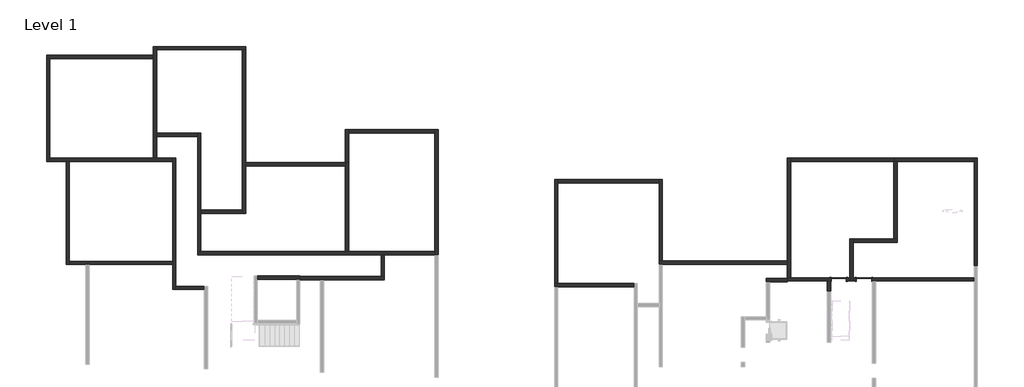
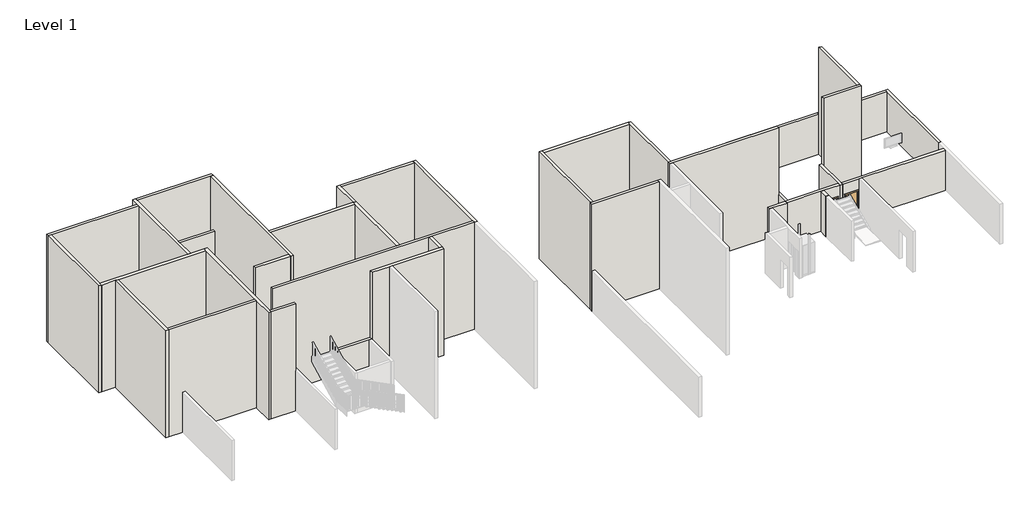
# One storey, part 2 of 3: 38 walls, 2 doors.
"""IFC4 building model written with IfcOpenShell, lengths in millimetres."""

import ifcopenshell
import ifcopenshell.guid

model = None  # the IFC model being written
_history = None  # IfcOwnerHistory: only IFC2X3 demands one
_inside = {}  # id of a spatial element -> (the spatial element, [elements in it])
_under = {}  # id of a project, library or spatial element -> (it, [spatial elements below it])
_declared = {}  # id of a project -> (the project, [libraries it declares])
_typed = {}  # id of a type object -> (the type object, [elements of that type])
_made_of = {}  # id of a material, layer set ... -> (it, [elements and type objects made of it])


def new_model(schema):
    """Start an empty IFC model of exactly this schema.

    Asked for "IFC4X3", IfcOpenShell would pick the latest addendum, in which some entities
    have other attributes; the version numbers below select the first issue.
    IFC2X3 requires an IfcOwnerHistory on every rooted entity: one is made here for all.
    """
    global model, _history
    if schema == "IFC4X3":
        model = ifcopenshell.file(schema_version=(4, 3, 0, 0))
    else:
        model = ifcopenshell.file(schema=schema)
    _inside.clear()
    _under.clear()
    _declared.clear()
    _typed.clear()
    _made_of.clear()
    _history = None
    if model.schema == "IFC2X3":
        org = make("IfcOrganization", Name="unknown")
        user = make(
            "IfcPersonAndOrganization",
            ThePerson=make("IfcPerson", FamilyName="unknown"),
            TheOrganization=org,
        )
        app = make(
            "IfcApplication",
            ApplicationDeveloper=org,
            Version="unknown",
            ApplicationFullName="unknown",
            ApplicationIdentifier="unknown",
        )
        _history = make(
            "IfcOwnerHistory",
            OwningUser=user,
            OwningApplication=app,
            ChangeAction="ADDED",
            CreationDate=0,
        )
    return model


def make(cls, **values):
    """One entity of the class cls with the attributes given. An attribute that is None is left unset."""
    return model.create_entity(
        cls, **{name: value for name, value in values.items() if value is not None}
    )


def rooted(cls, **values):
    """An entity with a GlobalId (a new one), such as an element, a storey or a relation."""
    return make(cls, GlobalId=ifcopenshell.guid.new(), OwnerHistory=_history, **values)


def si_unit(unit_type, name, prefix=None):
    """IfcSIUnit, for example si_unit("LENGTHUNIT", "METRE", prefix="MILLI")."""
    return make("IfcSIUnit", UnitType=unit_type, Prefix=prefix, Name=name)


def assignment(units):
    """IfcUnitAssignment: the units of a project."""
    return None if units is None else make("IfcUnitAssignment", Units=units)


def point(xyz):
    """IfcCartesianPoint."""
    return None if xyz is None else make("IfcCartesianPoint", Coordinates=xyz)


def direction(xyz):
    """IfcDirection."""
    return None if xyz is None else make("IfcDirection", DirectionRatios=xyz)


def frame(location, z_axis=None, x_axis=None):
    """IfcAxis2Placement3D, a coordinate frame: its origin and axes. An axis left out is left unset."""
    return make(
        "IfcAxis2Placement3D",
        Location=point(location),
        Axis=direction(z_axis),
        RefDirection=direction(x_axis),
    )


def origin():
    """The frame at (0, 0, 0) with its axes left unset."""
    return frame((0.0, 0.0, 0.0))


def origin_with_axes():
    """The frame at (0, 0, 0) with the z axis (0, 0, 1) and the x axis (1, 0, 0) written out."""
    return frame((0.0, 0.0, 0.0), z_axis=(0.0, 0.0, 1.0), x_axis=(1.0, 0.0, 0.0))


def place(relative_to, where):
    """IfcLocalPlacement: puts the frame where relative to a parent placement (None: the world)."""
    return make(
        "IfcLocalPlacement", PlacementRelTo=relative_to, RelativePlacement=where
    )


def context(
    kind, dimensions, precision=None, world=None, true_north=None, identifier=None
):
    """IfcGeometricRepresentationContext, for example the 3D "Model" context."""
    return make(
        "IfcGeometricRepresentationContext",
        ContextIdentifier=identifier,
        ContextType=kind,
        CoordinateSpaceDimension=dimensions,
        Precision=precision,
        WorldCoordinateSystem=world,
        TrueNorth=true_north,
    )


def project(units=None, contexts=None):
    """IfcProject with its units and contexts."""
    return rooted(
        "IfcProject",
        Name="project",
        RepresentationContexts=contexts,
        UnitsInContext=assignment(units),
    )


def spatial(cls, under=None, at=None, **own):
    """A site, building, storey or space (cls), placed at a placement, below another one or the project."""
    s = rooted(cls, ObjectPlacement=at, **own)
    if under is not None:
        _under.setdefault(under.id(), (under, []))[1].append(s)
    return s


def polyline(points):
    """IfcPolyline through the points."""
    return make("IfcPolyline", Points=[point(p) for p in points])


def outline(outer, holes=None, kind="AREA"):
    """IfcArbitraryClosedProfileDef: a profile drawn as a closed curve; with holes, ...WithVoids."""
    if holes is None:
        return make("IfcArbitraryClosedProfileDef", ProfileType=kind, OuterCurve=outer)
    return make(
        "IfcArbitraryProfileDefWithVoids",
        ProfileType=kind,
        OuterCurve=outer,
        InnerCurves=holes,
    )


def extrude(swept, where, along, depth):
    """IfcExtrudedAreaSolid: the profile swept, set in the frame where, extruded along a direction by depth."""
    return make(
        "IfcExtrudedAreaSolid",
        SweptArea=swept,
        Position=where,
        ExtrudedDirection=direction(along),
        Depth=depth,
    )


def faces_of(points, faces, orient=None, outer=None):
    """IfcFace entities. A face is a list of loops; a loop is a list of indices into points, from 0.

    orient and outer hold one flag for each loop. By default every Orientation is true, the
    first loop of a face is its IfcFaceOuterBound and the others are IfcFaceBound.
    """
    made = []
    for i, loops in enumerate(faces):
        bounds = []
        for j, loop in enumerate(loops):
            is_outer = j == 0 if outer is None else outer[i][j]
            bounds.append(
                make(
                    "IfcFaceOuterBound" if is_outer else "IfcFaceBound",
                    Bound=make("IfcPolyLoop", Polygon=[points[k] for k in loop]),
                    Orientation=True if orient is None else orient[i][j],
                )
            )
        made.append(make("IfcFace", Bounds=bounds))
    return made


def faceted_brep(points, faces, orient=None, outer=None, voids=None):
    """IfcFacetedBrep: a solid bounded by flat faces; with voids (closed shells), ...WithVoids."""
    shared = [point(p) for p in points]
    hull = make("IfcClosedShell", CfsFaces=faces_of(shared, faces, orient, outer))
    if voids is None:
        return make("IfcFacetedBrep", Outer=hull)
    return make(
        "IfcFacetedBrepWithVoids",
        Outer=hull,
        Voids=[
            make(cls, CfsFaces=faces_of(shared, fs, o, b)) for cls, fs, o, b in voids
        ],
    )


def shape(context_of_items, identifier, shape_type, items):
    """IfcShapeRepresentation: the items that make up one representation, for example the "Body"."""
    return make(
        "IfcShapeRepresentation",
        ContextOfItems=context_of_items,
        RepresentationIdentifier=identifier,
        RepresentationType=shape_type,
        Items=items,
    )


def source(mapping_origin, context_of_items, identifier, shape_type, items):
    """IfcRepresentationMap: a shape defined once, which mapped items show again and again."""
    return make(
        "IfcRepresentationMap",
        MappingOrigin=mapping_origin,
        MappedRepresentation=shape(context_of_items, identifier, shape_type, items),
    )


def transform(
    local_origin,
    x_axis=None,
    y_axis=None,
    z_axis=None,
    scale=None,
    scale2=None,
    scale3=None,
    uniform=True,
):
    """IfcCartesianTransformationOperator3D, or its non-uniform kind. x_axis, y_axis, z_axis: its Axis1, 2, 3."""
    if uniform:
        return make(
            "IfcCartesianTransformationOperator3D",
            Axis1=direction(x_axis),
            Axis2=direction(y_axis),
            LocalOrigin=point(local_origin),
            Scale=scale,
            Axis3=direction(z_axis),
        )
    return make(
        "IfcCartesianTransformationOperator3DnonUniform",
        Axis1=direction(x_axis),
        Axis2=direction(y_axis),
        LocalOrigin=point(local_origin),
        Scale=scale,
        Axis3=direction(z_axis),
        Scale2=scale2,
        Scale3=scale3,
    )


def mapped(mapping_source, mapping_target):
    """IfcMappedItem: shows the shape of a source again, moved by a transform."""
    return make(
        "IfcMappedItem", MappingSource=mapping_source, MappingTarget=mapping_target
    )


def made_of(thing, what):
    """Note that an element or type object is made of a material, layer set ...; save() writes the relation."""
    if what is not None:
        _made_of.setdefault(what.id(), (what, []))[1].append(thing)
    return thing


def element(
    cls,
    number,
    at=None,
    inside=None,
    cuts=None,
    type_object=None,
    material=None,
    context=None,
    identifier="Body",
    shape_type=None,
    held_by="IfcProductDefinitionShape",
    body=None,
    shapes=None,
    **own,
):
    """One element of the class cls, such as IfcWall. Its Tag is "e" and its number.

    at: its placement. inside: the storey or other place that contains it. cuts: it is an
    opening in that element (IfcRelVoidsElement). A single representation is given by context,
    identifier, shape_type and body (its items); several are given by shapes. held_by: the class
    of the entity that holds the representations. save() writes the other relations.
    """
    e = rooted(cls, Tag="e%d" % number, ObjectPlacement=at, **own)
    if body is not None:
        shapes = [shape(context, identifier, shape_type, body)]
    if shapes is not None:
        e.Representation = make(held_by, Representations=shapes)
    if inside is not None:
        _inside.setdefault(inside.id(), (inside, []))[1].append(e)
    if cuts is not None:
        rooted(
            "IfcRelVoidsElement", RelatingBuildingElement=cuts, RelatedOpeningElement=e
        )
    if type_object is not None:
        _typed.setdefault(type_object.id(), (type_object, []))[1].append(e)
    return made_of(e, material)


def aggregate(whole, parts):
    """IfcRelAggregates: a whole, such as a stair, and the parts it consists of."""
    return rooted("IfcRelAggregates", RelatingObject=whole, RelatedObjects=parts)


def save(model, path):
    """Write the relations noted so far, then the file.

    IfcRelAggregates (storeys below a building ...), IfcRelContainedInSpatialStructure (elements
    in a storey), IfcRelDefinesByType, IfcRelAssociatesMaterial and IfcRelDeclares: one each for
    every whole, place, type object, material and project.
    """
    for whole, parts in _under.values():
        aggregate(whole, parts)
    for where, things in _inside.values():
        rooted(
            "IfcRelContainedInSpatialStructure",
            RelatedElements=things,
            RelatingStructure=where,
        )
    for kind, things in _typed.values():
        rooted("IfcRelDefinesByType", RelatedObjects=things, RelatingType=kind)
    for what, things in _made_of.values():
        rooted("IfcRelAssociatesMaterial", RelatedObjects=things, RelatingMaterial=what)
    for by, libraries in _declared.values():
        rooted("IfcRelDeclares", RelatingContext=by, RelatedDefinitions=libraries)
    model.write(path)


def m_single_flush_0915_x_2134mm_727434cd(model_context):
    return source(origin(), model_context, "Body", "SweptSolid", [
        extrude(outline(polyline([(2210.0, -533.5), (0.0, -533.5), (0.0, -457.5), (2134.0, -457.5), (2134.0, 457.5), (0.0, 457.5), (0.0, 533.5), (2210.0, 533.5), (2210.0, -533.5)])), frame((0.0, -125.0, 0.0), z_axis=(0.0, 1.0, 0.0), x_axis=(0.0, 0.0, 1.0)), (0.0, 0.0, 1.0), 25.0),
        extrude(outline(polyline([(2210.0, 533.5), (2210.0, -533.5), (0.0, -533.5), (0.0, -457.5), (2134.0, -457.5), (2134.0, 457.5), (0.0, 457.5), (0.0, 533.5), (2210.0, 533.5)])), frame((0.0, 100.0, 0.0), z_axis=(0.0, 1.0, 0.0), x_axis=(0.0, 0.0, 1.0)), (0.0, 0.0, 1.0), 25.0),
        extrude(outline(polyline([(457.5, -49.0), (457.5, -100.0), (-457.5, -100.0), (-457.5, -49.0), (457.5, -49.0)])), origin_with_axes(), (0.0, 0.0, 1.0), 2134.0),
    ])


def m_single_flush_0915_x_2134mm_6a9e8738(model_context):
    return source(origin(), model_context, "Body", "SweptSolid", [
        extrude(outline(polyline([(2210.0, -533.5), (0.0, -533.5), (0.0, -457.5), (2134.0, -457.5), (2134.0, 457.5), (0.0, 457.5), (0.0, 533.5), (2210.0, 533.5), (2210.0, -533.5)])), frame((0.0, 100.0, 0.0), z_axis=(0.0, 1.0, 0.0), x_axis=(0.0, 0.0, 1.0)), (0.0, 0.0, 1.0), 25.0),
        extrude(outline(polyline([(2210.0, 533.5), (2210.0, -533.5), (0.0, -533.5), (0.0, -457.5), (2134.0, -457.5), (2134.0, 457.5), (0.0, 457.5), (0.0, 533.5), (2210.0, 533.5)])), frame((0.0, -125.0, 0.0), z_axis=(0.0, 1.0, 0.0), x_axis=(0.0, 0.0, 1.0)), (0.0, 0.0, 1.0), 25.0),
        extrude(outline(polyline([(457.5, 49.0), (-457.5, 49.0), (-457.5, 100.0), (457.5, 100.0), (457.5, 49.0)])), origin_with_axes(), (0.0, 0.0, 1.0), 2134.0),
    ])


model = new_model("IFC4")

# Units and contexts
model_context = context("Model", 3, world=origin())
ifc_project = project(units=[si_unit("LENGTHUNIT", "METRE", prefix="MILLI")], contexts=[model_context])

# Site, building, storey
site = spatial("IfcSite", under=ifc_project)
building = spatial("IfcBuilding", under=site)
storey = spatial("IfcBuildingStorey", under=building, Name="Level 1", Elevation=0.0)

# Doors
placement = place(None, origin())
m_single_flush_0915_x_2134mm_shape = m_single_flush_0915_x_2134mm_727434cd(model_context)
element("IfcDoor", 1, ObjectType="M_Single-Flush : 0915 x 2134mm", at=placement, inside=storey, context=model_context, shape_type="MappedRepresentation", body=[
    mapped(m_single_flush_0915_x_2134mm_shape, transform((23447.336337, 519.475628, 0.0), x_axis=(-1.0, 0.0, 0.0), y_axis=(0.0, -1.0, 0.0), z_axis=(0.0, 0.0, 1.0))),
])
m_single_flush_0915_x_2134mm_2_shape = m_single_flush_0915_x_2134mm_6a9e8738(model_context)
element("IfcDoor", 2, ObjectType="M_Single-Flush : 0915 x 2134mm", at=placement, inside=storey, context=model_context, shape_type="MappedRepresentation", body=[
    mapped(m_single_flush_0915_x_2134mm_2_shape, transform((21932.336337, 519.475628, 0.0), x_axis=(1.0, 0.0, 0.0), y_axis=(0.0, 1.0, 0.0), z_axis=(0.0, 0.0, 1.0))),
])

# Walls
element("IfcWall", 3, ObjectType="Generic - 200mm", at=placement, inside=storey, context=model_context, shape_type="Brep", body=[
    faceted_brep([(25249.836337, 7619.475628, 0.0), (25449.836337, 7619.475628, 0.0), (30068.3425199, 7619.475628, 0.0), (30068.3425199, 7619.475628, 3000.0), (25249.836337, 7619.475628, 3000.0), (25249.836337, 7819.475628, 0.0), (25249.836337, 7819.475628, 3000.0), (30068.3425199, 7819.475628, 3000.0), (30068.3425199, 7819.475628, 0.0)], [[[0, 1, 2, 3, 4]], [[5, 6, 7, 8]], [[2, 1, 0, 5, 8]], [[4, 3, 7, 6]], [[3, 2, 8, 7]], [[0, 4, 6, 5]]]),
])
element("IfcWall", 4, ObjectType="Generic - 200mm", at=placement, inside=storey, context=model_context, shape_type="Brep", body=[
    faceted_brep([(30068.3425199, 7819.475628, 0.0), (30068.3425199, 7619.475628, 0.0), (30068.3425199, 1319.475628, 0.0), (30068.3425199, 1319.475628, 3000.0), (30068.3425199, 7619.475628, 3000.0), (30068.3425199, 7819.475628, 3000.0), (30268.3425199, 7819.475628, 0.0), (30268.3425199, 7819.475628, 3000.0), (30268.3425199, 1319.475628, 3000.0), (30268.3425199, 1319.475628, 0.0), (30068.8612349, 1319.475628, 0.0), (30068.8612349, 1319.475628, 3000.0)], [[[0, 1, 2, 3, 4, 5]], [[6, 7, 8, 9]], [[2, 1, 0, 6, 9, 10]], [[3, 2, 10, 9, 8, 11]], [[5, 4, 3, 11, 8, 7]], [[0, 5, 7, 6]]]),
])
element("IfcWall", 5, ObjectType="Generic - 200mm", at=placement, inside=storey, context=model_context, shape_type="SweptSolid", body=[
    extrude(outline(polyline([(21449.836337, 419.475628), (21449.836337, -200.524372), (21249.836337, -200.524372), (21249.836337, 419.475628), (21449.836337, 419.475628)])), origin_with_axes(), (0.0, 0.0, 1.0), 3000.0),
])
element("IfcWall", 6, ObjectType="Generic - 200mm", at=placement, inside=storey, context=model_context, shape_type="SweptSolid", body=[
    extrude(outline(polyline([(25249.836337, 7619.475628), (19028.8612349, 7619.475628), (19028.8612349, 7819.475628), (25249.836337, 7819.475628), (25249.836337, 7619.475628)])), origin_with_axes(), (0.0, 0.0, 1.0), 3000.0),
])
element("IfcWall", 7, ObjectType="Generic - 200mm", at=placement, inside=storey, context=model_context, shape_type="Brep", body=[
    faceted_brep([(22789.836337, 419.475628, 0.0), (22789.836337, 619.475628, 0.0), (22789.836337, 2754.475628, 0.0), (22789.836337, 2954.475628, 0.0), (22789.836337, 2954.475628, 3000.0), (22789.836337, 619.475628, 3000.0), (22789.836337, 419.475628, 3000.0), (22589.836337, 419.475628, 0.0), (22589.836337, 419.475628, 3000.0), (22589.836337, 619.475628, 3000.0), (22589.836337, 2954.475628, 3000.0), (22589.836337, 2954.475628, 0.0), (22589.836337, 619.475628, 0.0)], [[[0, 1, 2, 3, 4, 5, 6]], [[7, 8, 9, 10, 11, 12]], [[3, 2, 1, 0, 7, 12, 11]], [[6, 5, 4, 10, 9, 8]], [[0, 6, 8, 7]], [[4, 3, 11, 10]]]),
])
element("IfcWall", 8, ObjectType="Generic - 200mm", at=placement, inside=storey, context=model_context, shape_type="Brep", body=[
    faceted_brep([(18828.8612349, 7819.475628, 0.0), (18828.8612349, 1619.475628, 0.0), (18828.8612349, 1419.475628, 0.0), (18828.8612349, 619.475628, 0.0), (18828.8612349, 619.475628, 3000.0), (18828.8612349, 7819.475628, 3000.0), (19028.8612349, 7819.475628, 0.0), (19028.8612349, 7819.475628, 3000.0), (19028.8612349, 7619.475628, 3000.0), (19028.8612349, 619.475628, 3000.0), (19028.8612349, 619.475628, 0.0), (19028.8612349, 7619.475628, 0.0)], [[[0, 1, 2, 3, 4, 5]], [[6, 7, 8, 9, 10, 11]], [[3, 2, 1, 0, 6, 11, 10]], [[5, 4, 9, 8, 7]], [[4, 3, 10, 9]], [[0, 5, 7, 6]]]),
])
element("IfcWall", 9, ObjectType="Generic - 200mm", at=placement, inside=storey, context=model_context, shape_type="Brep", body=[
    faceted_brep([(30068.8612349, 419.475628, 3000.0), (24148.8612349, 419.475628, 3000.0), (23948.8612349, 419.475628, 3000.0), (22789.836337, 419.475628, 3000.0), (22789.836337, 419.475628, 0.0), (22989.836337, 419.475628, 0.0), (22989.836337, 419.475628, 2134.0), (23904.836337, 419.475628, 2134.0), (23904.836337, 419.475628, 0.0), (23948.8612349, 419.475628, 0.0), (24148.8612349, 419.475628, 0.0), (30068.8612349, 419.475628, 0.0), (22789.836337, 619.475628, 3000.0), (30068.8612349, 619.475628, 3000.0), (30068.8612349, 619.475628, 0.0), (23904.836337, 619.475628, 0.0), (23904.836337, 619.475628, 2134.0), (22989.836337, 619.475628, 2134.0), (22989.836337, 619.475628, 0.0), (22789.836337, 619.475628, 0.0)], [[[0, 1, 2, 3, 4, 5, 6, 7, 8, 9, 10, 11]], [[12, 13, 14, 15, 16, 17, 18, 19]], [[14, 11, 10, 9, 8, 15]], [[4, 19, 18, 5]], [[3, 2, 1, 0, 13, 12]], [[0, 11, 14, 13]], [[4, 3, 12, 19]], [[17, 6, 5, 18]], [[7, 16, 15, 8]], [[16, 7, 6, 17]]]),
])
element("IfcWall", 10, ObjectType="Generic - 200mm", at=placement, inside=storey, context=model_context, shape_type="Brep", body=[
    faceted_brep([(18828.8612349, 579.475628, 0.0), (17570.6041014, 579.475628, 0.0), (17570.6041014, 579.475628, 3000.0), (18828.8612349, 579.475628, 3000.0), (18828.8612349, 379.475628, 0.0), (18828.8612349, 379.475628, 3000.0), (17770.6041014, 379.475628, 3000.0), (17570.6041014, 379.475628, 3000.0), (17570.6041014, 379.475628, 0.0), (17770.6041014, 379.475628, 0.0), (18828.8612349, 419.475628, 0.0), (18828.8612349, 419.475628, 3000.0)], [[[0, 1, 2, 3]], [[4, 5, 6, 7, 8, 9]], [[1, 0, 10, 4, 9, 8]], [[2, 1, 8, 7]], [[3, 2, 7, 6, 5, 11]], [[0, 3, 11, 5, 4, 10]]]),
])
element("IfcWall", 11, ObjectType="Generic - 200mm", at=placement, inside=storey, context=model_context, shape_type="Brep", body=[
    faceted_brep([(18828.8612349, 619.475628, 3000.0), (19028.8612349, 619.475628, 3000.0), (22589.836337, 619.475628, 3000.0), (22589.836337, 619.475628, 0.0), (22389.836337, 619.475628, 0.0), (22389.836337, 619.475628, 2134.0), (21474.836337, 619.475628, 2134.0), (21474.836337, 619.475628, 0.0), (19028.8612349, 619.475628, 0.0), (18828.8612349, 619.475628, 0.0), (22589.836337, 419.475628, 3000.0), (21449.836337, 419.475628, 3000.0), (21249.836337, 419.475628, 3000.0), (18828.8612349, 419.475628, 3000.0), (18828.8612349, 419.475628, 0.0), (21249.836337, 419.475628, 0.0), (21449.836337, 419.475628, 0.0), (21474.836337, 419.475628, 0.0), (21474.836337, 419.475628, 2134.0), (22389.836337, 419.475628, 2134.0), (22389.836337, 419.475628, 0.0), (22589.836337, 419.475628, 0.0), (18828.8612349, 579.475628, 0.0), (18828.8612349, 579.475628, 3000.0)], [[[0, 1, 2, 3, 4, 5, 6, 7, 8, 9]], [[10, 11, 12, 13, 14, 15, 16, 17, 18, 19, 20, 21]], [[3, 21, 20, 4]], [[14, 22, 9, 8, 7, 17, 16, 15]], [[2, 1, 0, 23, 13, 12, 11, 10]], [[0, 9, 22, 14, 13, 23]], [[3, 2, 10, 21]], [[19, 5, 4, 20]], [[6, 18, 17, 7]], [[18, 6, 5, 19]]]),
])
element("IfcWall", 12, ObjectType="Generic - 200mm", at=placement, inside=storey, context=model_context, shape_type="Brep", body=[
    faceted_brep([(22789.836337, 2754.475628, 0.0), (25449.836337, 2754.475628, 0.0), (25449.836337, 2754.475628, 8000.0), (22789.836337, 2754.475628, 8000.0), (22789.836337, 2954.475628, 0.0), (22789.836337, 2954.475628, 3000.0), (22789.836337, 2954.475628, 8000.0), (25249.836337, 2954.475628, 8000.0), (25449.836337, 2954.475628, 8000.0), (25449.836337, 2954.475628, 0.0), (25249.836337, 2954.475628, 0.0)], [[[0, 1, 2, 3]], [[4, 5, 6, 7, 8, 9, 10]], [[1, 0, 4, 10, 9]], [[3, 2, 8, 7, 6]], [[2, 1, 9, 8]], [[0, 3, 6, 5, 4]]]),
])
element("IfcWall", 13, ObjectType="Generic - 200mm", at=placement, inside=storey, context=model_context, shape_type="Brep", body=[
    faceted_brep([(25449.836337, 2954.475628, 0.0), (25449.836337, 7619.475628, 0.0), (25449.836337, 7619.475628, 8000.0), (25449.836337, 2954.475628, 8000.0), (25249.836337, 2954.475628, 0.0), (25249.836337, 2954.475628, 8000.0), (25249.836337, 7619.475628, 8000.0), (25249.836337, 7619.475628, 3000.0), (25249.836337, 7619.475628, 0.0)], [[[0, 1, 2, 3]], [[4, 5, 6, 7, 8]], [[1, 0, 4, 8]], [[3, 2, 6, 5]], [[0, 3, 5, 4]], [[2, 1, 8, 7, 6]]]),
])
element("IfcWall", 14, ObjectType="Generic - 200mm", at=placement, inside=storey, context=model_context, shape_type="Brep", body=[
    faceted_brep([(-10469.8304233, 720.8372871, 0.0), (-13026.101437, 720.8372871, 0.0), (-13026.101437, 720.8372871, 3000.0), (-10469.8304233, 720.8372871, 3000.0), (-10469.8304233, 520.8372871, 0.0), (-10469.8304233, 520.8372871, 3000.0), (-10669.8304233, 520.8372871, 3000.0), (-13026.101437, 520.8372871, 3000.0), (-13026.101437, 520.8372871, 0.0), (-10669.8304233, 520.8372871, 0.0), (-10469.8304233, 700.8372871, 0.0)], [[[0, 1, 2, 3]], [[4, 5, 6, 7, 8, 9]], [[1, 0, 10, 4, 9, 8]], [[3, 2, 7, 6, 5]], [[2, 1, 8, 7]], [[0, 3, 5, 4, 10]]]),
])
element("IfcWall", 15, ObjectType="Generic - 200mm", at=placement, inside=storey, context=model_context, shape_type="Brep", body=[
    faceted_brep([(-19089.8304233, 7812.8400285, 0.0), (-19089.8304233, 9112.8400285, 0.0), (-19089.8304233, 9312.8400285, 0.0), (-19089.8304233, 14340.8372871, 0.0), (-19089.8304233, 14540.8372871, 0.0), (-19089.8304233, 14540.8372871, 8000.0), (-19089.8304233, 14340.8372871, 8000.0), (-19089.8304233, 9312.8400285, 8000.0), (-19089.8304233, 9112.8400285, 8000.0), (-19089.8304233, 7812.8400285, 8000.0), (-19289.8304233, 7812.8400285, 0.0), (-19289.8304233, 7812.8400285, 8000.0), (-19289.8304233, 13812.8400285, 8000.0), (-19289.8304233, 14012.8400285, 8000.0), (-19289.8304233, 14540.8372871, 8000.0), (-19289.8304233, 14540.8372871, 0.0), (-19289.8304233, 14012.8400285, 0.0), (-19289.8304233, 13812.8400285, 0.0)], [[[0, 1, 2, 3, 4, 5, 6, 7, 8, 9]], [[10, 11, 12, 13, 14, 15, 16, 17]], [[4, 3, 2, 1, 0, 10, 17, 16, 15]], [[9, 8, 7, 6, 5, 14, 13, 12, 11]], [[5, 4, 15, 14]], [[0, 9, 11, 10]]]),
])
element("IfcWall", 16, ObjectType="Generic - 200mm", at=placement, inside=storey, context=model_context, shape_type="Brep", body=[
    faceted_brep([(9628.8612349, 279.9901881, 0.0), (5043.716007, 279.9901881, 0.0), (4843.716007, 279.9901881, 0.0), (4843.716007, 279.9901881, 8000.0), (5043.716007, 279.9901881, 8000.0), (9628.8612349, 279.9901881, 8000.0), (9628.8612349, 79.9901881, 0.0), (9628.8612349, 79.9901881, 8000.0), (4843.716007, 79.9901881, 8000.0), (4843.716007, 79.9901881, 3000.0), (4843.716007, 79.9901881, 0.0), (5043.716007, 79.9901881, 0.0)], [[[0, 1, 2, 3, 4, 5]], [[6, 7, 8, 9, 10, 11]], [[2, 1, 0, 6, 11, 10]], [[5, 4, 3, 8, 7]], [[0, 5, 7, 6]], [[2, 10, 9, 8, 3]]]),
])
element("IfcWall", 17, ObjectType="Generic - 200mm", at=placement, inside=storey, context=model_context, shape_type="Brep", body=[
    faceted_brep([(-13726.101437, 14540.8372871, 0.0), (-19089.8304233, 14540.8372871, 0.0), (-19089.8304233, 14540.8372871, 8000.0), (-13726.101437, 14540.8372871, 8000.0), (-13726.101437, 14340.8372871, 0.0), (-13726.101437, 14340.8372871, 8000.0), (-13926.101437, 14340.8372871, 8000.0), (-19089.8304233, 14340.8372871, 8000.0), (-19089.8304233, 14340.8372871, 0.0), (-13926.101437, 14340.8372871, 0.0)], [[[0, 1, 2, 3]], [[4, 5, 6, 7, 8, 9]], [[1, 0, 4, 9, 8]], [[3, 2, 7, 6, 5]], [[2, 1, 8, 7]], [[0, 3, 5, 4]]]),
])
element("IfcWall", 18, ObjectType="Generic - 200mm", at=placement, inside=storey, context=model_context, shape_type="Brep", body=[
    faceted_brep([(-25701.4369496, 13812.8400285, 0.0), (-25701.4369496, 7612.8400285, 0.0), (-25701.4369496, 7612.8400285, 8000.0), (-25701.4369496, 13812.8400285, 8000.0), (-25501.4369496, 13812.8400285, 0.0), (-25501.4369496, 13812.8400285, 8000.0), (-25501.4369496, 7812.8400285, 8000.0), (-25501.4369496, 7612.8400285, 8000.0), (-25501.4369496, 7612.8400285, 0.0), (-25501.4369496, 7812.8400285, 0.0)], [[[0, 1, 2, 3]], [[4, 5, 6, 7, 8, 9]], [[1, 0, 4, 9, 8]], [[3, 2, 7, 6, 5]], [[2, 1, 8, 7]], [[0, 3, 5, 4]]]),
])
element("IfcWall", 19, ObjectType="Generic - 200mm", at=placement, inside=storey, context=model_context, shape_type="Brep", body=[
    faceted_brep([(-25501.4369496, 7612.8400285, 0.0), (-24523.9741722, 7612.8400285, 0.0), (-24323.9741722, 7612.8400285, 0.0), (-18123.9741722, 7612.8400285, 0.0), (-18123.9741722, 7612.8400285, 8000.0), (-24323.9741722, 7612.8400285, 8000.0), (-24523.9741722, 7612.8400285, 8000.0), (-25501.4369496, 7612.8400285, 8000.0), (-25501.4369496, 7812.8400285, 0.0), (-25501.4369496, 7812.8400285, 8000.0), (-19289.8304233, 7812.8400285, 8000.0), (-19089.8304233, 7812.8400285, 8000.0), (-18123.9741722, 7812.8400285, 8000.0), (-18123.9741722, 7812.8400285, 0.0), (-19089.8304233, 7812.8400285, 0.0), (-19289.8304233, 7812.8400285, 0.0)], [[[0, 1, 2, 3, 4, 5, 6, 7]], [[8, 9, 10, 11, 12, 13, 14, 15]], [[3, 2, 1, 0, 8, 15, 14, 13]], [[7, 6, 5, 4, 12, 11, 10, 9]], [[0, 7, 9, 8]], [[4, 3, 13, 12]]]),
])
element("IfcWall", 20, ObjectType="Generic - 200mm", at=placement, inside=storey, context=model_context, shape_type="Brep", body=[
    faceted_brep([(-19289.8304233, 14012.8400285, 0.0), (-25701.4369496, 14012.8400285, 0.0), (-25701.4369496, 14012.8400285, 8000.0), (-19289.8304233, 14012.8400285, 8000.0), (-19289.8304233, 13812.8400285, 0.0), (-19289.8304233, 13812.8400285, 8000.0), (-25501.4369496, 13812.8400285, 8000.0), (-25701.4369496, 13812.8400285, 8000.0), (-25701.4369496, 13812.8400285, 0.0), (-25501.4369496, 13812.8400285, 0.0)], [[[0, 1, 2, 3]], [[4, 5, 6, 7, 8, 9]], [[1, 0, 4, 9, 8]], [[3, 2, 7, 6, 5]], [[2, 1, 8, 7]], [[0, 3, 5, 4]]]),
])
element("IfcWall", 21, ObjectType="Generic - 200mm", at=placement, inside=storey, context=model_context, shape_type="Brep", body=[
    faceted_brep([(-24523.9741722, 7612.8400285, 0.0), (-24523.9741722, 1412.8400285, 0.0), (-24523.9741722, 1412.8400285, 8000.0), (-24523.9741722, 7612.8400285, 8000.0), (-24323.9741722, 7612.8400285, 0.0), (-24323.9741722, 7612.8400285, 8000.0), (-24323.9741722, 1612.8400285, 8000.0), (-24323.9741722, 1412.8400285, 8000.0), (-24323.9741722, 1412.8400285, 0.0), (-24323.9741722, 1612.8400285, 0.0)], [[[0, 1, 2, 3]], [[4, 5, 6, 7, 8, 9]], [[1, 0, 4, 9, 8]], [[3, 2, 7, 6, 5]], [[0, 3, 5, 4]], [[2, 1, 8, 7]]]),
])
element("IfcWall", 22, ObjectType="Generic - 200mm", at=placement, inside=storey, context=model_context, shape_type="Brep", body=[
    faceted_brep([(-24323.9741722, 1412.8400285, 0.0), (-23346.5113948, 1412.8400285, 0.0), (-23146.5113948, 1412.8400285, 0.0), (-18123.9741722, 1412.8400285, 0.0), (-18123.9741722, 1412.8400285, 8000.0), (-24323.9741722, 1412.8400285, 8000.0), (-24323.9741722, 1612.8400285, 0.0), (-24323.9741722, 1612.8400285, 8000.0), (-18123.9741722, 1612.8400285, 8000.0), (-18123.9741722, 1612.8400285, 0.0)], [[[0, 1, 2, 3, 4, 5]], [[6, 7, 8, 9]], [[3, 2, 1, 0, 6, 9]], [[5, 4, 8, 7]], [[0, 5, 7, 6]], [[4, 3, 9, 8]]]),
])
element("IfcWall", 23, ObjectType="Generic - 200mm", at=placement, inside=storey, context=model_context, shape_type="Brep", body=[
    faceted_brep([(-19089.8304233, 9112.8400285, 0.0), (-16623.9741722, 9112.8400285, 0.0), (-16623.9741722, 9112.8400285, 8000.0), (-19089.8304233, 9112.8400285, 8000.0), (-19089.8304233, 9312.8400285, 0.0), (-19089.8304233, 9312.8400285, 8000.0), (-16623.9741722, 9312.8400285, 8000.0), (-16623.9741722, 9312.8400285, 3000.0), (-16623.9741722, 9312.8400285, 0.0)], [[[0, 1, 2, 3]], [[4, 5, 6, 7, 8]], [[1, 0, 4, 8]], [[3, 2, 6, 5]], [[0, 3, 5, 4]], [[2, 1, 8, 7, 6]]]),
])
element("IfcWall", 24, ObjectType="Generic - 200mm", at=placement, inside=storey, context=model_context, shape_type="Brep", body=[
    faceted_brep([(-18123.9741722, 7812.8400285, 0.0), (-18123.9741722, 7612.8400285, 0.0), (-18123.9741722, 1612.8400285, 0.0), (-18123.9741722, 1412.8400285, 0.0), (-18123.9741722, -87.1599715, 0.0), (-18123.9741722, -87.1599715, 8000.0), (-18123.9741722, 1412.8400285, 8000.0), (-18123.9741722, 1612.8400285, 8000.0), (-18123.9741722, 7612.8400285, 8000.0), (-18123.9741722, 7812.8400285, 8000.0), (-17923.9741722, 7812.8400285, 0.0), (-17923.9741722, 7812.8400285, 8000.0), (-17923.9741722, 112.8400285, 8000.0), (-17923.9741722, -87.1599715, 8000.0), (-17923.9741722, -87.1599715, 0.0), (-17923.9741722, 112.8400285, 0.0)], [[[0, 1, 2, 3, 4, 5, 6, 7, 8, 9]], [[10, 11, 12, 13, 14, 15]], [[4, 3, 2, 1, 0, 10, 15, 14]], [[9, 8, 7, 6, 5, 13, 12, 11]], [[0, 9, 11, 10]], [[5, 4, 14, 13]]]),
])
element("IfcWall", 25, ObjectType="Generic - 200mm", at=placement, inside=storey, context=model_context, shape_type="Brep", body=[
    faceted_brep([(-7730.3449834, 7540.8372871, 0.0), (-7730.3449834, 7340.8372871, 0.0), (-7730.3449834, 2200.8372871, 0.0), (-7730.3449834, 2200.8372871, 8000.0), (-7730.3449834, 7340.8372871, 8000.0), (-7730.3449834, 7540.8372871, 8000.0), (-7530.3449834, 7540.8372871, 0.0), (-7530.3449834, 7540.8372871, 8000.0), (-7530.3449834, 2200.8372871, 8000.0), (-7530.3449834, 2200.8372871, 0.0)], [[[0, 1, 2, 3, 4, 5]], [[6, 7, 8, 9]], [[2, 1, 0, 6, 9]], [[5, 4, 3, 8, 7]], [[0, 5, 7, 6]], [[3, 2, 9, 8]]]),
])
element("IfcWall", 26, ObjectType="Generic - 200mm", at=placement, inside=storey, context=model_context, shape_type="Brep", body=[
    faceted_brep([(-17923.9741722, -87.1599715, 0.0), (-16213.9741722, -87.1599715, 0.0), (-16213.9741722, -87.1599715, 8000.0), (-17923.9741722, -87.1599715, 8000.0), (-17923.9741722, 112.8400285, 0.0), (-17923.9741722, 112.8400285, 8000.0), (-16213.9741722, 112.8400285, 8000.0), (-16213.9741722, 112.8400285, 3000.0), (-16213.9741722, 112.8400285, 0.0)], [[[0, 1, 2, 3]], [[4, 5, 6, 7, 8]], [[1, 0, 4, 8]], [[3, 2, 6, 5]], [[0, 3, 5, 4]], [[2, 1, 8, 7, 6]]]),
])
element("IfcWall", 27, ObjectType="Generic - 200mm", at=placement, inside=storey, context=model_context, shape_type="Brep", body=[
    faceted_brep([(-16423.9741722, 2200.8372871, 0.0), (-16423.9741722, 4500.8372871, 0.0), (-16423.9741722, 4700.8372871, 0.0), (-16423.9741722, 9312.8400285, 0.0), (-16423.9741722, 9312.8400285, 3000.0), (-16423.9741722, 2200.8372871, 3000.0), (-16623.9741722, 2200.8372871, 0.0), (-16623.9741722, 2200.8372871, 3000.0), (-16623.9741722, 9312.8400285, 3000.0), (-16623.9741722, 9312.8400285, 0.0), (-16623.9741722, 9112.8400285, 0.0)], [[[0, 1, 2, 3, 4, 5]], [[6, 7, 8, 9, 10]], [[3, 2, 1, 0, 6, 10, 9]], [[5, 4, 8, 7]], [[0, 5, 7, 6]], [[4, 3, 9, 8]]]),
])
element("IfcWall", 28, ObjectType="Generic - 200mm", at=placement, inside=storey, context=model_context, shape_type="SweptSolid", body=[
    extrude(outline(polyline([(-13726.101437, 7540.8372871), (-7730.3449834, 7540.8372871), (-7730.3449834, 7340.8372871), (-13726.101437, 7340.8372871), (-13726.101437, 7540.8372871)])), origin_with_axes(), (0.0, 0.0, 1.0), 8000.0),
])
element("IfcWall", 29, ObjectType="Generic - 200mm", at=placement, inside=storey, context=model_context, shape_type="Brep", body=[
    faceted_brep([(-16623.9741722, 2000.8372871, 0.0), (-5590.3449834, 2000.8372871, 0.0), (-5390.3449834, 2000.8372871, 0.0), (-2360.3449834, 2000.8372871, 0.0), (-2350.3449834, 2000.8372871, 0.0), (-2350.3449834, 2000.8372871, 8000.0), (-2360.3449834, 2000.8372871, 8000.0), (-5390.3449834, 2000.8372871, 8000.0), (-5590.3449834, 2000.8372871, 8000.0), (-16623.9741722, 2000.8372871, 8000.0), (-16623.9741722, 2200.8372871, 0.0), (-16623.9741722, 2200.8372871, 3000.0), (-16623.9741722, 2200.8372871, 8000.0), (-7730.3449834, 2200.8372871, 8000.0), (-7530.3449834, 2200.8372871, 8000.0), (-2350.3449834, 2200.8372871, 8000.0), (-2350.3449834, 2200.8372871, 0.0), (-7530.3449834, 2200.8372871, 0.0), (-7730.3449834, 2200.8372871, 0.0), (-16423.9741722, 2200.8372871, 0.0)], [[[0, 1, 2, 3, 4, 5, 6, 7, 8, 9]], [[10, 11, 12, 13, 14, 15, 16, 17, 18, 19]], [[4, 3, 2, 1, 0, 10, 19, 18, 17, 16]], [[9, 8, 7, 6, 5, 15, 14, 13, 12]], [[0, 9, 12, 11, 10]], [[5, 4, 16, 15]]]),
])
element("IfcWall", 30, ObjectType="Generic - 200mm", at=placement, inside=storey, context=model_context, shape_type="Brep", body=[
    faceted_brep([(-5390.3449834, 700.8372871, 0.0), (-5590.3449834, 700.8372871, 0.0), (-10469.8304233, 700.8372871, 0.0), (-10469.8304233, 700.8372871, 8000.0), (-5590.3449834, 700.8372871, 8000.0), (-5390.3449834, 700.8372871, 8000.0), (-5390.3449834, 500.8372871, 0.0), (-5390.3449834, 500.8372871, 8000.0), (-9030.3629108, 500.8372871, 8000.0), (-9230.3629108, 500.8372871, 8000.0), (-10469.8304233, 500.8372871, 8000.0), (-10469.8304233, 500.8372871, 0.0), (-9230.3629108, 500.8372871, 0.0), (-9030.3629108, 500.8372871, 0.0), (-10469.8304233, 520.8372871, 0.0)], [[[0, 1, 2, 3, 4, 5]], [[6, 7, 8, 9, 10, 11, 12, 13]], [[2, 1, 0, 6, 13, 12, 11, 14]], [[5, 4, 3, 10, 9, 8, 7]], [[3, 2, 14, 11, 10]], [[0, 5, 7, 6]]]),
])
element("IfcWall", 31, ObjectType="Generic - 200mm", at=placement, inside=storey, context=model_context, shape_type="Brep", body=[
    faceted_brep([(-2350.3449834, 9540.8372871, 0.0), (-2350.3449834, 9340.8372871, 0.0), (-2350.3449834, 2200.8372871, 0.0), (-2350.3449834, 2000.8372871, 0.0), (-2350.3449834, 2000.8372871, 8000.0), (-2350.3449834, 2200.8372871, 8000.0), (-2350.3449834, 9340.8372871, 8000.0), (-2350.3449834, 9540.8372871, 8000.0), (-2150.3449834, 9540.8372871, 0.0), (-2150.3449834, 9540.8372871, 8000.0), (-2150.3449834, 2000.8372871, 8000.0), (-2150.3449834, 2000.8372871, 0.0), (-2160.3449834, 2000.8372871, 0.0), (-2160.3449834, 2000.8372871, 8000.0)], [[[0, 1, 2, 3, 4, 5, 6, 7]], [[8, 9, 10, 11]], [[3, 2, 1, 0, 8, 11, 12]], [[7, 6, 5, 4, 13, 10, 9]], [[0, 7, 9, 8]], [[4, 3, 12, 11, 10, 13]]]),
])
element("IfcWall", 32, ObjectType="Generic - 200mm", at=placement, inside=storey, context=model_context, shape_type="Brep", body=[
    faceted_brep([(11128.8612349, 1419.475628, 0.0), (11328.8612349, 1419.475628, 0.0), (18828.8612349, 1419.475628, 0.0), (18828.8612349, 1419.475628, 8000.0), (11328.8612349, 1419.475628, 8000.0), (11128.8612349, 1419.475628, 8000.0), (11128.8612349, 1619.475628, 0.0), (11128.8612349, 1619.475628, 8000.0), (11328.8612349, 1619.475628, 8000.0), (18828.8612349, 1619.475628, 8000.0), (18828.8612349, 1619.475628, 0.0), (11328.8612349, 1619.475628, 0.0)], [[[0, 1, 2, 3, 4, 5]], [[6, 7, 8, 9, 10, 11]], [[2, 1, 0, 6, 11, 10]], [[5, 4, 3, 9, 8, 7]], [[3, 2, 10, 9]], [[0, 5, 7, 6]]]),
])
element("IfcWall", 33, ObjectType="Generic - 200mm", at=placement, inside=storey, context=model_context, shape_type="Brep", body=[
    faceted_brep([(5043.716007, 279.9901881, 0.0), (5043.716007, 6319.475628, 0.0), (5043.716007, 6519.475628, 0.0), (5043.716007, 6519.475628, 8000.0), (5043.716007, 6319.475628, 8000.0), (5043.716007, 279.9901881, 8000.0), (4843.716007, 279.9901881, 0.0), (4843.716007, 279.9901881, 8000.0), (4843.716007, 6519.475628, 8000.0), (4843.716007, 6519.475628, 0.0)], [[[0, 1, 2, 3, 4, 5]], [[6, 7, 8, 9]], [[2, 1, 0, 6, 9]], [[5, 4, 3, 8, 7]], [[0, 5, 7, 6]], [[3, 2, 9, 8]]]),
])
element("IfcWall", 34, ObjectType="Generic - 200mm", at=placement, inside=storey, context=model_context, shape_type="Brep", body=[
    faceted_brep([(11328.8612349, 1619.475628, 0.0), (11328.8612349, 6519.475628, 0.0), (11328.8612349, 6519.475628, 8000.0), (11328.8612349, 1619.475628, 8000.0), (11128.8612349, 1619.475628, 0.0), (11128.8612349, 1619.475628, 8000.0), (11128.8612349, 6319.475628, 8000.0), (11128.8612349, 6519.475628, 8000.0), (11128.8612349, 6519.475628, 0.0), (11128.8612349, 6319.475628, 0.0)], [[[0, 1, 2, 3]], [[4, 5, 6, 7, 8, 9]], [[1, 0, 4, 9, 8]], [[3, 2, 7, 6, 5]], [[0, 3, 5, 4]], [[2, 1, 8, 7]]]),
])
element("IfcWall", 35, ObjectType="Generic - 200mm", at=placement, inside=storey, context=model_context, shape_type="SweptSolid", body=[
    extrude(outline(polyline([(5043.716007, 6519.475628), (11128.8612349, 6519.475628), (11128.8612349, 6319.475628), (5043.716007, 6319.475628), (5043.716007, 6519.475628)])), origin_with_axes(), (0.0, 0.0, 1.0), 8000.0),
])
element("IfcWall", 36, ObjectType="Generic - 200mm", at=placement, inside=storey, context=model_context, shape_type="Brep", body=[
    faceted_brep([(-13926.101437, 14340.8372871, 0.0), (-13926.101437, 4700.8372871, 0.0), (-13926.101437, 4500.8372871, 0.0), (-13926.101437, 4500.8372871, 8000.0), (-13926.101437, 4700.8372871, 8000.0), (-13926.101437, 14340.8372871, 8000.0), (-13726.101437, 14340.8372871, 0.0), (-13726.101437, 14340.8372871, 8000.0), (-13726.101437, 7540.8372871, 8000.0), (-13726.101437, 7340.8372871, 8000.0), (-13726.101437, 4500.8372871, 8000.0), (-13726.101437, 4500.8372871, 0.0), (-13726.101437, 7340.8372871, 0.0), (-13726.101437, 7540.8372871, 0.0)], [[[0, 1, 2, 3, 4, 5]], [[6, 7, 8, 9, 10, 11, 12, 13]], [[2, 1, 0, 6, 13, 12, 11]], [[5, 4, 3, 10, 9, 8, 7]], [[3, 2, 11, 10]], [[0, 5, 7, 6]]]),
])
element("IfcWall", 37, ObjectType="Generic - 200mm", at=placement, inside=storey, context=model_context, shape_type="SweptSolid", body=[
    extrude(outline(polyline([(-16423.9741722, 4700.8372871), (-13926.101437, 4700.8372871), (-13926.101437, 4500.8372871), (-16423.9741722, 4500.8372871), (-16423.9741722, 4700.8372871)])), origin_with_axes(), (0.0, 0.0, 1.0), 8000.0),
])
element("IfcWall", 38, ObjectType="Generic - 200mm", at=placement, inside=storey, context=model_context, shape_type="SweptSolid", body=[
    extrude(outline(polyline([(-5390.3449834, 2000.8372871), (-5390.3449834, 700.8372871), (-5590.3449834, 700.8372871), (-5590.3449834, 2000.8372871), (-5390.3449834, 2000.8372871)])), origin_with_axes(), (0.0, 0.0, 1.0), 8000.0),
])
element("IfcWall", 39, ObjectType="Generic - 200mm", at=placement, inside=storey, context=model_context, shape_type="Brep", body=[
    faceted_brep([(-7530.3449834, 7540.8372871, 0.0), (-7530.3449834, 9340.8372871, 0.0), (-7530.3449834, 9540.8372871, 0.0), (-7530.3449834, 9540.8372871, 8000.0), (-7530.3449834, 9340.8372871, 8000.0), (-7530.3449834, 7540.8372871, 8000.0), (-7730.3449834, 7540.8372871, 0.0), (-7730.3449834, 7540.8372871, 8000.0), (-7730.3449834, 9540.8372871, 8000.0), (-7730.3449834, 9540.8372871, 0.0)], [[[0, 1, 2, 3, 4, 5]], [[6, 7, 8, 9]], [[2, 1, 0, 6, 9]], [[5, 4, 3, 8, 7]], [[0, 5, 7, 6]], [[3, 2, 9, 8]]]),
])
element("IfcWall", 40, ObjectType="Generic - 200mm", at=placement, inside=storey, context=model_context, shape_type="SweptSolid", body=[
    extrude(outline(polyline([(-2350.3449834, 9340.8372871), (-7530.3449834, 9340.8372871), (-7530.3449834, 9540.8372871), (-2350.3449834, 9540.8372871), (-2350.3449834, 9340.8372871)])), origin_with_axes(), (0.0, 0.0, 1.0), 8000.0),
])

save(model, "model.ifc")

# Revit data of these elements
# Type "M_Single-Flush : 0915 x 2134mm"
#   Type Mark = "20"
#   Construction Type Id = "MDOOR"
#   Analytic Construction = "Metal"
#   Thickness = 5.1 cm
#   Thermal Resistance (R) = 0.270117 (m²·K)/W
#   Heat Transfer Coefficient (U) = 3.7021 W/(m²·K)
#   Height = 213.4 cm
#   Trim Projection Ext = 2.5 cm
#   Trim Projection Int = 2.5 cm
#   Trim Width = 7.6 cm
#   Width = 91.5 cm
#   Define Thermal Properties by = 1
#   Define Thermal Properties by = 1
#   Door Material = Door - Panel
#   Frame Material = Door - Frame
#   Visual Light Transmittance = 0
#   Solar Heat Gain Coefficient = 0
#   Function = (empty or 0)
#   Wall Closure = (empty or 0)
# Type "Generic - 200mm"
#   Layers, outside or top first: 20 cm no material (function 1)
# Elements 1, 2 (IfcDoor, "M_Single-Flush : 0915 x 2134mm")
#   Phase Created = New Construction
#   Materials on its faces: "Door - Frame", "Door - Panel"
# Elements 3, 4, 5, 6, 7, 8, 9, 10, 11, 14, 27 (IfcWall, "Generic - 200mm")
#   Top Offset = 0 cm
#   Base Offset = 0 cm
#   wall height = 300 cm
#   Phase Created = New Construction
#   Base Constraint = Level 1
#   Top Constraint = Level 2
#   Materials on its faces: "Default Wall"
# Elements 12, 13, 15, 16, 17, 18, 19, 20, 21, 22, 23, 24, 25, 26, 28, 29, 30, 31, 32, 33, 34, 35, 36, 37, 38, 39, 40 (IfcWall, "Generic - 200mm")
#   Top Offset = 0 cm
#   Base Offset = 0 cm
#   Unconnected Height = 800 cm
#   wall height = 800 cm
#   Phase Created = New Construction
#   Base Constraint = Level 1
#   Materials on its faces: "Default Wall"
# Materials
#   "Door - Panel": class "Wood", colour RGB 210 159 95, transparency 0, Cost = 0
#   "Door - Frame": class "Miscellaneous", colour RGB 118 70 51, transparency 0, Cost = 0
#   "Default Wall": class "Miscellaneous", colour RGB 128 128 128, transparency 0, Cost = 0
